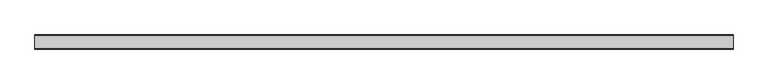
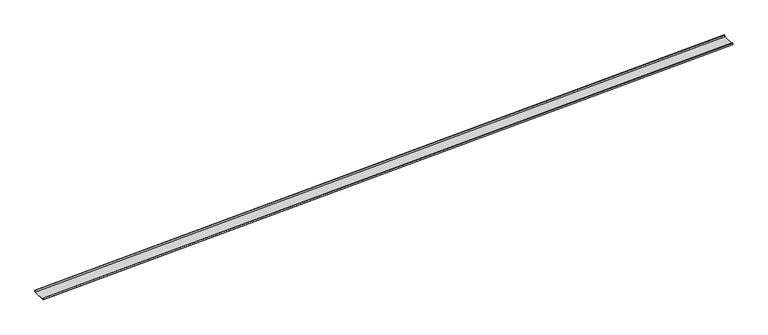
"""IFC4 building model written with IfcOpenShell, lengths in millimetres: proxy geometry, Generic Models 2:Generic Models 2:310765:Generic Models 2:310765 : Generic Models 2:Generic Models 2:310765:82 : Generic Models 2:Generic Models 2:310765:Generic Models 2:310765 : Generic Models 2:Generic Models 2:310765:300385."""

from ifc_helpers import new_model, si_unit, frame, origin, place, context, project, spatial, polyline, outline, extrude, source, transform, mapped, element, save


def generic_models_73a410d6(model_context):
    return source(origin(), model_context, "Body", "SweptSolid", [
        extrude(outline(polyline([(1.5875, 0.0), (1.5875, 50.8), (407.9875, 50.8), (407.9875, 1.5874999), (396.875, 1.5874999), (396.875, 11.1124999), (398.4625, 11.1124999), (398.4625, 3.175), (406.4, 3.175), (406.4, 49.2124999), (3.175, 49.2124999), (3.175, -1.5875), (-14.2875, -1.5875), (-14.2875, 9.525), (-12.7, 9.525), (-12.7, 0.0), (1.5875, 0.0)])), frame((558205.3611715, -578114.072634, 3910.7299065), z_axis=(0.9991330730923568, 0.0, 0.041630544712067834), x_axis=(0.0, -1.0, 0.0)), (0.0, 0.0, 1.0), 20863.1091694),
    ])


if __name__ == "__main__":
    model = new_model("IFC4")
    model_context = context("Model", 3, world=origin())
    ifc_project = project(units=[si_unit("LENGTHUNIT", "METRE", prefix="MILLI")], contexts=[model_context])
    site = spatial("IfcSite", under=ifc_project)
    building = spatial("IfcBuilding", under=site)
    placement = place(None, origin())
    generic_models_shape = generic_models_73a410d6(model_context)
    element("IfcBuildingElementProxy", 1, Name="Generic Models 2:Generic Models 2:310765:Generic Models 2:310765 : Generic Models 2:Generic Models 2:310765:82 : Generic Models 2:Generic Models 2:310765:Generic Models 2:310765 : Generic Models 2:Generic Models 2:310765:300385", ObjectType="Generic Models 2:Generic Models 2:310765:Generic Models 2:310765 : Generic Models 2:Generic Models 2:310765:82 : Generic Models 2:Generic Models 2:310765:Generic Models 2:310765 : Generic Models 2:Generic Models 2:310765:300385", at=placement, inside=building, context=model_context, shape_type="MappedRepresentation", body=[
        mapped(generic_models_shape, transform((0.0, 0.0, 0.0), x_axis=(1.0, 0.0, 0.0), y_axis=(0.0, 1.0, 0.0), z_axis=(0.0, 0.0, 1.0))),
    ])
    save(model, "model.ifc")

# Revit data of these elements
# Type "Generic Models 2:Generic Models 2:310765:Generic Models 2:310765 : Generic Models 2:Generic Models 2:310765:82 : Generic Models 2:Generic Models 2:310765:Generic Models 2:310765 : Generic Models 2:Generic Models 2:310765:300385"
#   NameOverride = "Generic Models 2:Generic Models 2:310765:Generic Models 2:310765 : Generic Models 2:Generic Models 2:310765:300385"
#   ObjectTypeOverride = "Generic Models 2:310765 : Generic Models 2:Generic Models 2:310765"
#   Reference = "Generic Models 2"
#   Tag = "300385"
# Element 1 (IfcBuildingElementProxy, "Generic Models 2:Generic Models 2:310765:Generic Models 2:310765 : Generic Models 2:Generic Models 2:310765:82 : Generic Models 2:Generic Models 2:310765:Generic Models 2:310765 : Generic Models 2:Generic Models 2:310765:300385")
#   Materials on its faces: "STRUCTURAL STANDING SEAM SHEET METAL ROOFING - BATTENLOK - COLOR T.B.D."
# Materials
#   "STRUCTURAL STANDING SEAM SHEET METAL ROOFING - BATTENLOK - COLOR T.B.D.": class "Generic", colour RGB 120 120 120, transparency 0, Cost = 0
